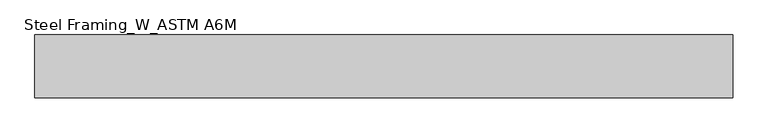
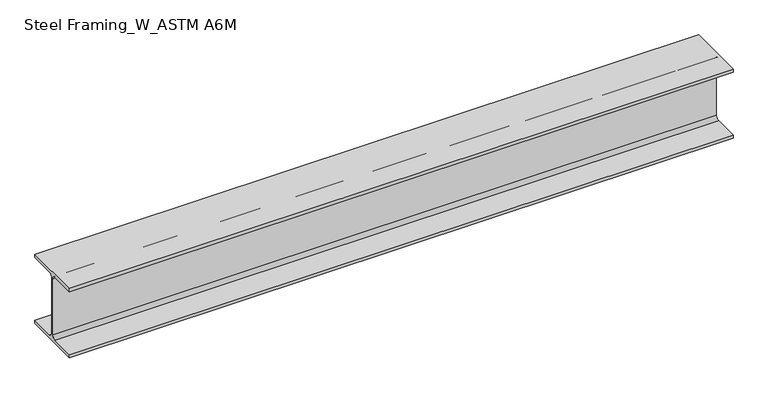
"""IFC4 building model written with IfcOpenShell, lengths in millimetres: beam geometry, Steel Framing_W_ASTM A6M : H_SB_AR_S02_W250x49.1_RCG1."""

from ifc_helpers import new_model, si_unit, point, frame, frame_2d, origin, place, context, project, spatial, polyline, circle_curve, trimmed, segment, composite_curve, outline, extrude, source, transform, mapped, element, save


def steel_framing_w_astm_a6m_3b9d56c5(model_context):
    return source(origin(), model_context, "Body", "SweptSolid", [
        extrude(outline(composite_curve([segment(polyline([(101.0, -112.5), (101.0, -123.5), (-101.0, -123.5), (-101.0, -112.5), (-16.385, -112.5)]), True, "CONTINUOUS"), segment(trimmed(circle_curve(frame_2d((-16.385, -99.8)), 12.7), [point((-16.385, -112.5))], [point((-3.685, -99.8))], True, "CARTESIAN"), True, "CONTINUOUS"), segment(polyline([(-3.685, -99.8), (-3.685, 99.8)]), True, "CONTINUOUS"), segment(trimmed(circle_curve(frame_2d((-16.385, 99.8)), 12.7), [point((-3.685, 99.8))], [point((-16.385, 112.5))], True, "CARTESIAN"), True, "CONTINUOUS"), segment(polyline([(-16.385, 112.5), (-101.0, 112.5), (-101.0, 123.5), (101.0, 123.5), (101.0, 112.5), (16.385, 112.5)]), True, "CONTINUOUS"), segment(trimmed(circle_curve(frame_2d((16.385, 99.8)), 12.7), [point((16.385, 112.5))], [point((3.685, 99.8))], True, "CARTESIAN"), True, "CONTINUOUS"), segment(polyline([(3.685, 99.8), (3.685, -99.8)]), True, "CONTINUOUS"), segment(trimmed(circle_curve(frame_2d((16.385, -99.8)), 12.7), [point((3.685, -99.8))], [point((16.385, -112.5))], True, "CARTESIAN"), True, "CONTINUOUS"), segment(polyline([(16.385, -112.5), (101.0, -112.5)]), True, "CONTINUOUS")], self_intersect=False)), frame((-984.1, 0.0, 0.0), z_axis=(1.0, 0.0, 0.0), x_axis=(0.0, 1.0, 0.0)), (0.0, 0.0, 1.0), 2240.3),
    ])


if __name__ == "__main__":
    model = new_model("IFC4")
    model_context = context("Model", 3, world=origin())
    ifc_project = project(units=[si_unit("LENGTHUNIT", "METRE", prefix="MILLI")], contexts=[model_context])
    site = spatial("IfcSite", under=ifc_project)
    building = spatial("IfcBuilding", under=site)
    placement = place(None, origin())
    steel_framing_w_astm_a6m_shape = steel_framing_w_astm_a6m_3b9d56c5(model_context)
    element("IfcBeam", 1, ObjectType="Steel Framing_W_ASTM A6M : H_SB_AR_S02_W250x49.1_RCG1", at=placement, inside=building, context=model_context, shape_type="MappedRepresentation", body=[
        mapped(steel_framing_w_astm_a6m_shape, transform((0.0, 0.0, 0.0), x_axis=(1.0, 0.0, 0.0), y_axis=(0.0, 1.0, 0.0), z_axis=(0.0, 0.0, 1.0))),
    ])
    save(model, "model.ifc")

# Revit data of these elements
# Type "Steel Framing_W_ASTM A6M : H_SB_AR_S02_W250x49.1_RCG1"
#   Section Name Key = "W10x33"
#   Width = 20.2 cm
#   Web Thickness = 0.737 cm
#   Web Fillet = 1.27 cm
#   Warping Constant = 212000.0 cm⁶
#   Torsional Moment of Inertia = 24.30 cm⁴
#   Section Area = 62.6 cm²
#   Plastic Modulus weak axis = 229.0 cm³
#   Plastic Modulus strong axis = 636.0 cm³
#   Perimeter = 1.27 m²/m
#   Nominal Weight = 49.10 kgf/m
#   Moment of Inertia weak axis = 1520.00 cm⁴
#   Moment of Inertia strong axis = 7120.00 cm⁴
#   Height = 24.7 cm
#   Flange Thickness = 1.1 cm
#   Elastic Modulus weak axis = 151.0 cm³
#   Elastic Modulus strong axis = 574.0 cm³
#   Centroid Vertical = 12.35 cm
#   Centroid Horizontal = 10.1 cm
#   Length [instance default] = 1500 mm
#   Structural Material [instance default] = Steel, 45-345
#   Bolt Spacing = 0
#   Assembly Code = ""
# Element 1 (IfcBeam, "Steel Framing_W_ASTM A6M : H_SB_AR_S02_W250x49.1_RCG1")
#   Materials on its faces: "Steel, 45-345"
# Materials
#   "Steel, 45-345": class "Metal", colour RGB 189 187 185, transparency 0, Description = "Steel 345 MPa", Cost = 0
